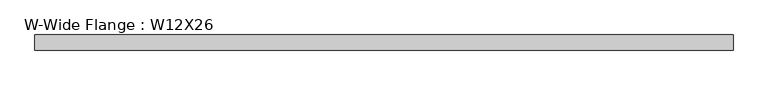
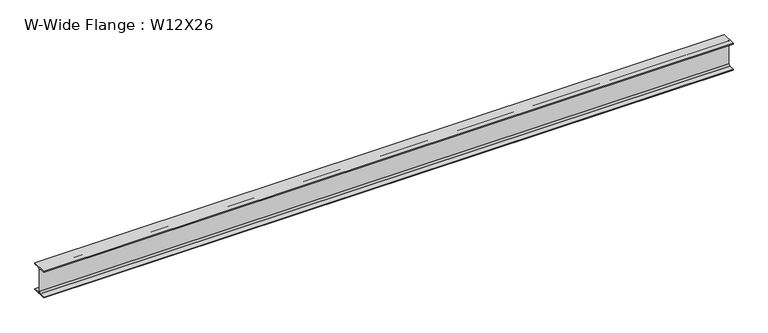
"""IFC4 building model written with IfcOpenShell, lengths in millimetres: beam geometry, W-Wide Flange : W12X26."""

from ifc_helpers import new_model, si_unit, point, frame, frame_2d, origin, place, context, project, spatial, polyline, circle_curve, trimmed, segment, composite_curve, outline, extrude, source, transform, mapped, element, save


def w_wide_flange_w12x26_c187b6f9(model_context):
    return source(origin(), model_context, "Body", "SweptSolid", [
        extrude(outline(composite_curve([segment(polyline([(82.423, -145.288), (82.423, -154.94), (-82.423, -154.94), (-82.423, -145.288), (-20.2565, -145.288)]), True, "CONTINUOUS"), segment(trimmed(circle_curve(frame_2d((-20.2565, -127.9525)), 17.3355), [point((-20.2565, -145.288))], [point((-2.921, -127.9525))], True, "CARTESIAN"), True, "CONTINUOUS"), segment(polyline([(-2.921, -127.9525), (-2.921, 127.9525)]), True, "CONTINUOUS"), segment(trimmed(circle_curve(frame_2d((-20.2565, 127.9525)), 17.3355), [point((-2.921, 127.9525))], [point((-20.2565, 145.288))], True, "CARTESIAN"), True, "CONTINUOUS"), segment(polyline([(-20.2565, 145.288), (-82.423, 145.288), (-82.423, 154.94), (82.423, 154.94), (82.423, 145.288), (20.2565, 145.288)]), True, "CONTINUOUS"), segment(trimmed(circle_curve(frame_2d((20.2565, 127.9525)), 17.3355), [point((20.2565, 145.288))], [point((2.921, 127.9525))], True, "CARTESIAN"), True, "CONTINUOUS"), segment(polyline([(2.921, 127.9525), (2.921, -127.9525)]), True, "CONTINUOUS"), segment(trimmed(circle_curve(frame_2d((20.2565, -127.9525)), 17.3355), [point((2.921, -127.9525))], [point((20.2565, -145.288))], True, "CARTESIAN"), True, "CONTINUOUS"), segment(polyline([(20.2565, -145.288), (82.423, -145.288)]), True, "CONTINUOUS")], self_intersect=False)), frame((-3797.3, 0.0, 0.0), z_axis=(1.0, 0.0, 0.0), x_axis=(0.0, 1.0, 0.0)), (0.0, 0.0, 1.0), 7594.6),
    ])


if __name__ == "__main__":
    model = new_model("IFC4")
    model_context = context("Model", 3, world=origin())
    ifc_project = project(units=[si_unit("LENGTHUNIT", "METRE", prefix="MILLI")], contexts=[model_context])
    site = spatial("IfcSite", under=ifc_project)
    building = spatial("IfcBuilding", under=site)
    placement = place(None, origin())
    w_wide_flange_w12x26_shape = w_wide_flange_w12x26_c187b6f9(model_context)
    element("IfcBeam", 1, ObjectType="W-Wide Flange : W12X26", at=placement, inside=building, context=model_context, shape_type="MappedRepresentation", body=[
        mapped(w_wide_flange_w12x26_shape, transform((0.0, 0.0, 0.0), x_axis=(1.0, 0.0, 0.0), y_axis=(0.0, 1.0, 0.0), z_axis=(0.0, 0.0, 1.0))),
    ])
    save(model, "model.ifc")

# Revit data of these elements
# Type "W-Wide Flange : W12X26"
#   Assembly Code = "B10"
#   W = 26
#   Length [instance default] = 5' - 0"
#   bf = 0' - 6.49"
#   d = 1' - 0.2"
#   k = 0' - 1 1/16"
#   k2 = 0' - 0.6825"
#   tf = 0' - 0.38"
#   tw = 0' - 0.23"
#   A = 0.053125 SF
#   Structural Material [instance default] = Steel ASTM A992
# Element 1 (IfcBeam, "W-Wide Flange : W12X26")
#   Materials on its faces: "Steel ASTM A992"
# Materials
#   "Steel ASTM A992": class "Metal", colour RGB 199 199 199, transparency 0, Description = "Structural steel 50ksi", Cost = 0
